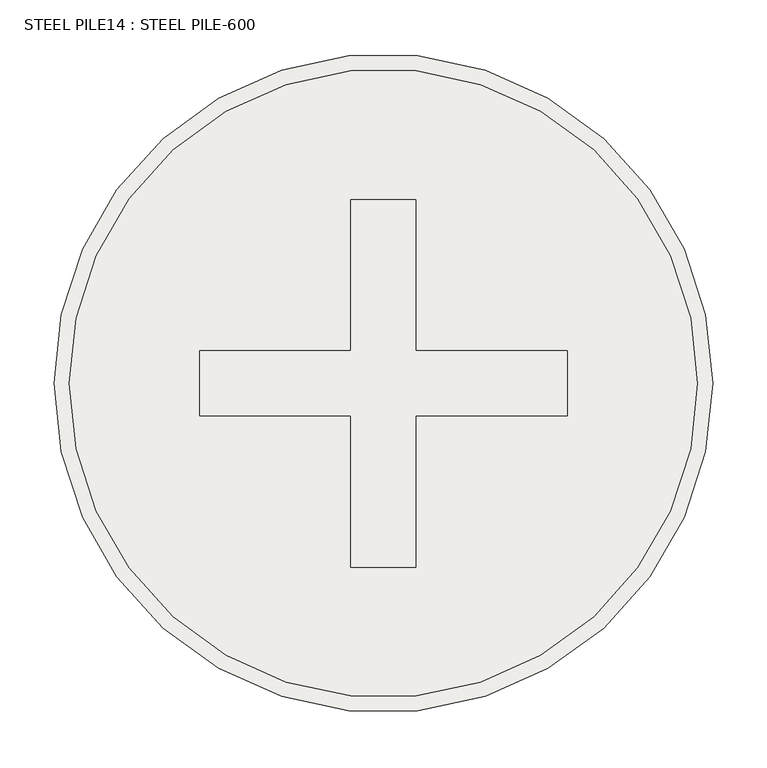
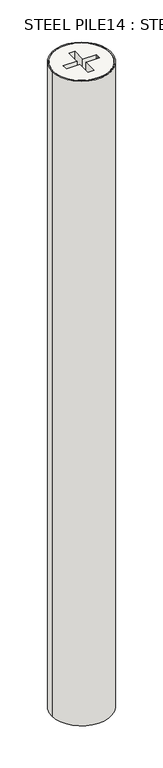
"""IFC4 building model written with IfcOpenShell, lengths in millimetres: slab geometry, STEEL PILE14 : STEEL PILE-600."""

from ifc_helpers import new_model, si_unit, point, frame, frame_2d, origin, place, context, project, spatial, circle_curve, trimmed, segment, composite_curve, outline, extrude, source, transform, mapped, element, save
from ifc_brep_helpers import plane_surface, cylinder_surface, advanced_brep


def steel_pile14_steel_pile_600_49f1fcfe(model_context):
    return source(origin(), model_context, "Body", "SolidModel", [
        advanced_brep(
        [(8709.5, 25499.5208589, 150.0), (9290.5, 25499.5208589, 150.0), (8970.0, 25469.5208589, 150.0), (8830.0, 25469.5208589, 150.0), (8830.0, 25499.5208589, 150.0), (8830.0, 25529.5208589, 150.0), (8970.0, 25529.5208589, 150.0), (8970.0, 25669.5208589, 150.0), (9030.0, 25669.5208589, 150.0), (9030.0, 25529.5208589, 150.0), (9170.0, 25529.5208589, 150.0), (9170.0, 25499.5208589, 150.0), (9170.0, 25469.5208589, 150.0), (9030.0, 25469.5208589, 150.0), (9030.0, 25329.5208589, 150.0), (8970.0, 25329.5208589, 150.0), (8709.5, 25499.5208589, -1850.0), (9290.5, 25499.5208589, -1850.0), (8830.0, 25469.5208589, -160.0), (8970.0, 25469.5208589, -160.0), (8970.0, 25329.5208589, -160.0), (9030.0, 25329.5208589, -160.0), (9030.0, 25469.5208589, -160.0), (9170.0, 25469.5208589, -160.0), (9170.0, 25499.5208589, -160.0), (9170.0, 25529.5208589, -160.0), (9030.0, 25529.5208589, -160.0), (9030.0, 25669.5208589, -160.0), (8970.0, 25669.5208589, -160.0), (8970.0, 25529.5208589, -160.0), (8830.0, 25529.5208589, -160.0), (8830.0, 25499.5208589, -160.0)],
        [
            (0, 1, circle_curve(frame((9000.0, 25499.5208589, 150.0), z_axis=(0.0, 0.0, 1.0), x_axis=(1.0, 0.0, 0.0)), 290.5)),
            (1, 0, circle_curve(frame((9000.0, 25499.5208589, 150.0), z_axis=(0.0, 0.0, 1.0), x_axis=(1.0, 0.0, 0.0)), 290.5)),
            (2, 3),
            (3, 4),
            (4, 5),
            (5, 6),
            (6, 7),
            (7, 8),
            (8, 9),
            (9, 10),
            (10, 11),
            (11, 12),
            (12, 13),
            (13, 14),
            (14, 15),
            (15, 2),
            (16, 17, circle_curve(frame((9000.0, 25499.5208589, -1850.0), z_axis=(0.0, 0.0, -1.0), x_axis=(1.0, 0.0, 0.0)), 290.5)),
            (17, 16, circle_curve(frame((9000.0, 25499.5208589, -1850.0), z_axis=(0.0, 0.0, -1.0), x_axis=(1.0, 0.0, 0.0)), 290.5)),
            (0, 16),
            (17, 1),
            (18, 19),
            (19, 20),
            (20, 21),
            (21, 22),
            (22, 23),
            (23, 24),
            (24, 25),
            (25, 26),
            (26, 27),
            (27, 28),
            (28, 29),
            (29, 30),
            (30, 31),
            (31, 18),
            (18, 3),
            (2, 19),
            (15, 20),
            (14, 21),
            (13, 22),
            (12, 23),
            (11, 24),
            (10, 25),
            (9, 26),
            (8, 27),
            (7, 28),
            (6, 29),
            (5, 30),
            (4, 31),
        ],
        [
            plane_surface(frame((9290.5, 25499.5208589, 150.0), z_axis=(0.0, 0.0, 1.0), x_axis=(0.0, 1.0, 0.0))),
            plane_surface(frame((9290.5, 25499.5208589, -1850.0), z_axis=(0.0, 0.0, -1.0), x_axis=(0.0, -1.0, 0.0))),
            cylinder_surface(frame((9000.0, 25499.5208589, -1850.0), z_axis=(0.0, 0.0, 1.0), x_axis=(1.0, 0.0, 0.0)), 290.5),
            plane_surface(frame((8830.0, 25469.5208589, -160.0), z_axis=(0.0, 0.0, 1.0), x_axis=(-1.0, 0.0, 0.0))),
            plane_surface(frame((8830.0, 25469.5208589, 160.0), z_axis=(0.0, 1.0, 0.0), x_axis=(0.0, 0.0, -1.0))),
            plane_surface(frame((8970.0, 25469.5208589, 160.0), z_axis=(1.0, 0.0, 0.0), x_axis=(0.0, 0.0, -1.0))),
            plane_surface(frame((8970.0, 25329.5208589, 160.0), z_axis=(0.0, 1.0, 0.0), x_axis=(0.0, 0.0, -1.0))),
            plane_surface(frame((9030.0, 25329.5208589, 160.0), z_axis=(-1.0, 0.0, 0.0), x_axis=(0.0, 0.0, -1.0))),
            plane_surface(frame((9030.0, 25469.5208589, 160.0), z_axis=(0.0, 1.0, 0.0), x_axis=(0.0, 0.0, -1.0))),
            plane_surface(frame((9170.0, 25469.5208589, 160.0), z_axis=(-1.0, 0.0, 0.0), x_axis=(0.0, 0.0, -1.0))),
            plane_surface(frame((9170.0, 25499.5208589, 160.0), z_axis=(-1.0, 0.0, 0.0), x_axis=(0.0, 0.0, -1.0))),
            plane_surface(frame((9170.0, 25529.5208589, 160.0), z_axis=(0.0, -1.0, 0.0), x_axis=(0.0, 0.0, -1.0))),
            plane_surface(frame((9030.0, 25529.5208589, 160.0), z_axis=(-1.0, 0.0, 0.0), x_axis=(0.0, 0.0, -1.0))),
            plane_surface(frame((9030.0, 25669.5208589, 160.0), z_axis=(0.0, -1.0, 0.0), x_axis=(0.0, 0.0, -1.0))),
            plane_surface(frame((8970.0, 25669.5208589, 160.0), z_axis=(1.0, 0.0, 0.0), x_axis=(0.0, 0.0, -1.0))),
            plane_surface(frame((8970.0, 25529.5208589, 160.0), z_axis=(0.0, -1.0, 0.0), x_axis=(0.0, 0.0, -1.0))),
            plane_surface(frame((8830.0, 25529.5208589, 160.0), z_axis=(1.0, 0.0, 0.0), x_axis=(0.0, 0.0, -1.0))),
            plane_surface(frame((8830.0, 25499.5208589, 160.0), z_axis=(1.0, 0.0, 0.0), x_axis=(0.0, 0.0, -1.0))),
        ],
        [
            (0, [[1, 2], [3, 4, 5, 6, 7, 8, 9, 10, 11, 12, 13, 14, 15, 16]]),
            (1, [[17, 18]]),
            (2, [[-1, 19, -18, 20]]),
            (2, [[-2, -20, -17, -19]]),
            (3, [[21, 22, 23, 24, 25, 26, 27, 28, 29, 30, 31, 32, 33, 34]]),
            (4, [[-21, 35, -3, 36]]),
            (5, [[-22, -36, -16, 37]]),
            (6, [[-23, -37, -15, 38]]),
            (7, [[-24, -38, -14, 39]]),
            (8, [[-25, -39, -13, 40]]),
            (9, [[-26, -40, -12, 41]]),
            (10, [[-27, -41, -11, 42]]),
            (11, [[-28, -42, -10, 43]]),
            (12, [[-29, -43, -9, 44]]),
            (13, [[-30, -44, -8, 45]]),
            (14, [[-31, -45, -7, 46]]),
            (15, [[-32, -46, -6, 47]]),
            (16, [[-33, -47, -5, 48]]),
            (17, [[-34, -48, -4, -35]]),
        ],
    ),
        extrude(outline(composite_curve([segment(trimmed(circle_curve(frame_2d((9000.0, 25499.5208589)), 304.5), [point((8695.5, 25499.5208589))], [point((9304.5, 25499.5208589))], False, "CARTESIAN"), True, "CONTINUOUS"), segment(trimmed(circle_curve(frame_2d((9000.0, 25499.5208589)), 304.5), [point((9304.5, 25499.5208589))], [point((8695.5, 25499.5208589))], False, "CARTESIAN"), True, "CONTINUOUS")], self_intersect=False), holes=[composite_curve([segment(trimmed(circle_curve(frame_2d((9000.0, 25499.5208589)), 290.5), [point((8709.5, 25499.5208589))], [point((9290.5, 25499.5208589))], True, "CARTESIAN"), True, "CONTINUOUS"), segment(trimmed(circle_curve(frame_2d((9000.0, 25499.5208589)), 290.5), [point((9290.5, 25499.5208589))], [point((8709.5, 25499.5208589))], True, "CARTESIAN"), True, "CONTINUOUS")], self_intersect=False)]), frame((0.0, 0.0, -6850.0), z_axis=(0.0, 0.0, 1.0), x_axis=(1.0, 0.0, 0.0)), (0.0, 0.0, 1.0), 7000.0),
    ])


if __name__ == "__main__":
    model = new_model("IFC4")
    model_context = context("Model", 3, world=origin())
    ifc_project = project(units=[si_unit("LENGTHUNIT", "METRE", prefix="MILLI")], contexts=[model_context])
    site = spatial("IfcSite", under=ifc_project)
    building = spatial("IfcBuilding", under=site)
    placement = place(None, origin())
    steel_pile14_steel_pile_600_shape = steel_pile14_steel_pile_600_49f1fcfe(model_context)
    element("IfcSlab", 1, ObjectType="STEEL PILE14 : STEEL PILE-600", at=placement, inside=building, context=model_context, shape_type="MappedRepresentation", body=[
        mapped(steel_pile14_steel_pile_600_shape, transform((0.0, 0.0, 0.0), x_axis=(1.0, 0.0, 0.0), y_axis=(0.0, 1.0, 0.0), z_axis=(0.0, 0.0, 1.0))),
    ])
    save(model, "model.ifc")
